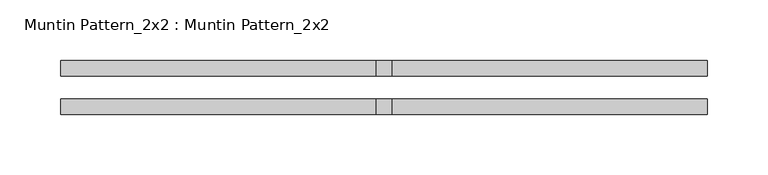
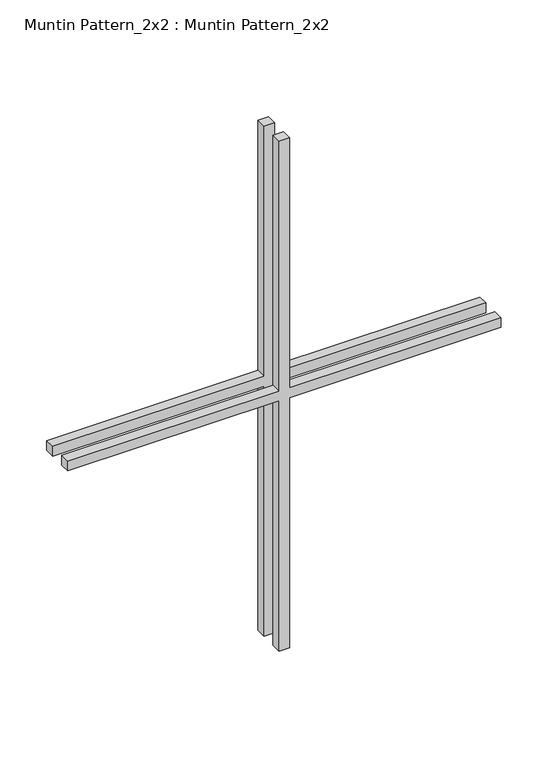
"""IFC4 building model written with IfcOpenShell, lengths in millimetres: proxy geometry, Muntin Pattern_2x2 : Muntin Pattern_2x2."""

from ifc_helpers import new_model, si_unit, frame, origin, place, context, project, spatial, polyline, outline, extrude, source, transform, mapped, element, save


def muntin_pattern_2x2_muntin_pattern_2x2_d95f8610(model_context):
    return source(origin(), model_context, "Body", "SweptSolid", [
        extrude(outline(polyline([(338.1375, -6.35), (338.1375, -266.7), (325.4375, -266.7), (325.4375, -6.35), (0.0, -6.35), (0.0, 6.35), (325.4375, 6.35), (325.4375, 266.7), (338.1375, 266.7), (338.1375, 6.35), (663.575, 6.35), (663.575, -6.35), (338.1375, -6.35)])), frame((0.0, 9.525, 0.0), z_axis=(0.0, 1.0, 0.0), x_axis=(0.0, 0.0, 1.0)), (0.0, 0.0, 1.0), 12.7),
        extrude(outline(polyline([(338.1375, -6.35), (338.1375, -266.7), (325.4375, -266.7), (325.4375, -6.35), (0.0, -6.35), (0.0, 6.35), (325.4375, 6.35), (325.4375, 266.7), (338.1375, 266.7), (338.1375, 6.35), (663.575, 6.35), (663.575, -6.35), (338.1375, -6.35)])), frame((0.0, -22.225, 0.0), z_axis=(0.0, 1.0, 0.0), x_axis=(0.0, 0.0, 1.0)), (0.0, 0.0, 1.0), 12.7),
    ])


if __name__ == "__main__":
    model = new_model("IFC4")
    model_context = context("Model", 3, world=origin())
    ifc_project = project(units=[si_unit("LENGTHUNIT", "METRE", prefix="MILLI")], contexts=[model_context])
    site = spatial("IfcSite", under=ifc_project)
    building = spatial("IfcBuilding", under=site)
    placement = place(None, origin())
    muntin_pattern_2x2_muntin_pattern_2x2_shape = muntin_pattern_2x2_muntin_pattern_2x2_d95f8610(model_context)
    element("IfcBuildingElementProxy", 1, Name="Muntin Pattern_2x2 : Muntin Pattern_2x2", ObjectType="Muntin Pattern_2x2 : Muntin Pattern_2x2", at=placement, inside=building, context=model_context, shape_type="MappedRepresentation", body=[
        mapped(muntin_pattern_2x2_muntin_pattern_2x2_shape, transform((0.0, 0.0, 0.0), x_axis=(1.0, 0.0, 0.0), y_axis=(0.0, 1.0, 0.0), z_axis=(0.0, 0.0, 1.0))),
    ])
    save(model, "model.ifc")

# Revit data of these elements
# Type "Muntin Pattern_2x2 : Muntin Pattern_2x2"
#   Width [instance default] = 4' - 0"
#   Thickness = 0' - 0 1/2"
#   Height [instance default] = 4' - 0"
#   Distance = 0' - 0 3/4"
#   Interior Material [instance default] = none
#   Exterior Material [instance default] = none
#   Default Elevation = 0
# Element 1 (IfcBuildingElementProxy, "Muntin Pattern_2x2 : Muntin Pattern_2x2")
#   Width = 1' - 9"
#   Height = 2' - 2 1/8"
#   Interior Material = Wood - Stained
#   Exterior Material = Clad - White
#   Materials on its faces: "Clad - White", "Wood - Stained"
# Materials
#   "Clad - White": class "Wood", colour RGB 242 242 238, transparency 0, Cost = 0
#   "Wood - Stained": class "Wood", colour RGB 224 178 126, transparency 0, Cost = 0
